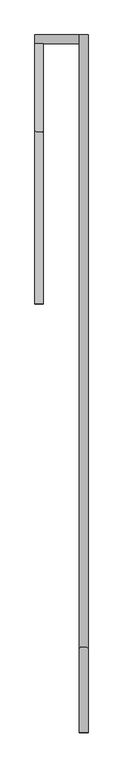
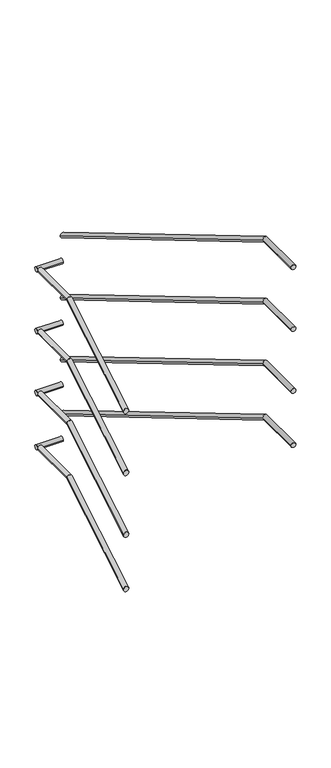
"""IFC4 building model written with IfcOpenShell, lengths in millimetres: railing geometry."""

import ifcopenshell
import ifcopenshell.guid

model = None  # the IFC model being written
_history = None  # IfcOwnerHistory: only IFC2X3 demands one
_inside = {}  # id of a spatial element -> (the spatial element, [elements in it])
_under = {}  # id of a project, library or spatial element -> (it, [spatial elements below it])
_declared = {}  # id of a project -> (the project, [libraries it declares])
_typed = {}  # id of a type object -> (the type object, [elements of that type])
_made_of = {}  # id of a material, layer set ... -> (it, [elements and type objects made of it])


def new_model(schema):
    """Start an empty IFC model of exactly this schema.

    Asked for "IFC4X3", IfcOpenShell would pick the latest addendum, in which some entities
    have other attributes; the version numbers below select the first issue.
    IFC2X3 requires an IfcOwnerHistory on every rooted entity: one is made here for all.
    """
    global model, _history
    if schema == "IFC4X3":
        model = ifcopenshell.file(schema_version=(4, 3, 0, 0))
    else:
        model = ifcopenshell.file(schema=schema)
    _inside.clear()
    _under.clear()
    _declared.clear()
    _typed.clear()
    _made_of.clear()
    _history = None
    if model.schema == "IFC2X3":
        org = make("IfcOrganization", Name="unknown")
        user = make(
            "IfcPersonAndOrganization",
            ThePerson=make("IfcPerson", FamilyName="unknown"),
            TheOrganization=org,
        )
        app = make(
            "IfcApplication",
            ApplicationDeveloper=org,
            Version="unknown",
            ApplicationFullName="unknown",
            ApplicationIdentifier="unknown",
        )
        _history = make(
            "IfcOwnerHistory",
            OwningUser=user,
            OwningApplication=app,
            ChangeAction="ADDED",
            CreationDate=0,
        )
    return model


def make(cls, **values):
    """One entity of the class cls with the attributes given. An attribute that is None is left unset."""
    return model.create_entity(
        cls, **{name: value for name, value in values.items() if value is not None}
    )


def rooted(cls, **values):
    """An entity with a GlobalId (a new one), such as an element, a storey or a relation."""
    return make(cls, GlobalId=ifcopenshell.guid.new(), OwnerHistory=_history, **values)


def si_unit(unit_type, name, prefix=None):
    """IfcSIUnit, for example si_unit("LENGTHUNIT", "METRE", prefix="MILLI")."""
    return make("IfcSIUnit", UnitType=unit_type, Prefix=prefix, Name=name)


def assignment(units):
    """IfcUnitAssignment: the units of a project."""
    return None if units is None else make("IfcUnitAssignment", Units=units)


def point(xyz):
    """IfcCartesianPoint."""
    return None if xyz is None else make("IfcCartesianPoint", Coordinates=xyz)


def direction(xyz):
    """IfcDirection."""
    return None if xyz is None else make("IfcDirection", DirectionRatios=xyz)


def frame(location, z_axis=None, x_axis=None):
    """IfcAxis2Placement3D, a coordinate frame: its origin and axes. An axis left out is left unset."""
    return make(
        "IfcAxis2Placement3D",
        Location=point(location),
        Axis=direction(z_axis),
        RefDirection=direction(x_axis),
    )


def origin():
    """The frame at (0, 0, 0) with its axes left unset."""
    return frame((0.0, 0.0, 0.0))


def place(relative_to, where):
    """IfcLocalPlacement: puts the frame where relative to a parent placement (None: the world)."""
    return make(
        "IfcLocalPlacement", PlacementRelTo=relative_to, RelativePlacement=where
    )


def context(
    kind, dimensions, precision=None, world=None, true_north=None, identifier=None
):
    """IfcGeometricRepresentationContext, for example the 3D "Model" context."""
    return make(
        "IfcGeometricRepresentationContext",
        ContextIdentifier=identifier,
        ContextType=kind,
        CoordinateSpaceDimension=dimensions,
        Precision=precision,
        WorldCoordinateSystem=world,
        TrueNorth=true_north,
    )


def project(units=None, contexts=None):
    """IfcProject with its units and contexts."""
    return rooted(
        "IfcProject",
        Name="project",
        RepresentationContexts=contexts,
        UnitsInContext=assignment(units),
    )


def spatial(cls, under=None, at=None, **own):
    """A site, building, storey or space (cls), placed at a placement, below another one or the project."""
    s = rooted(cls, ObjectPlacement=at, **own)
    if under is not None:
        _under.setdefault(under.id(), (under, []))[1].append(s)
    return s


def circle_curve(where, radius):
    """IfcCircle in the frame where."""
    return make("IfcCircle", Position=where, Radius=radius)


def ellipse_curve(where, semi_axis1, semi_axis2):
    """IfcEllipse in the frame where."""
    return make(
        "IfcEllipse", Position=where, SemiAxis1=semi_axis1, SemiAxis2=semi_axis2
    )


def shape(context_of_items, identifier, shape_type, items):
    """IfcShapeRepresentation: the items that make up one representation, for example the "Body"."""
    return make(
        "IfcShapeRepresentation",
        ContextOfItems=context_of_items,
        RepresentationIdentifier=identifier,
        RepresentationType=shape_type,
        Items=items,
    )


def source(mapping_origin, context_of_items, identifier, shape_type, items):
    """IfcRepresentationMap: a shape defined once, which mapped items show again and again."""
    return make(
        "IfcRepresentationMap",
        MappingOrigin=mapping_origin,
        MappedRepresentation=shape(context_of_items, identifier, shape_type, items),
    )


def transform(
    local_origin,
    x_axis=None,
    y_axis=None,
    z_axis=None,
    scale=None,
    scale2=None,
    scale3=None,
    uniform=True,
):
    """IfcCartesianTransformationOperator3D, or its non-uniform kind. x_axis, y_axis, z_axis: its Axis1, 2, 3."""
    if uniform:
        return make(
            "IfcCartesianTransformationOperator3D",
            Axis1=direction(x_axis),
            Axis2=direction(y_axis),
            LocalOrigin=point(local_origin),
            Scale=scale,
            Axis3=direction(z_axis),
        )
    return make(
        "IfcCartesianTransformationOperator3DnonUniform",
        Axis1=direction(x_axis),
        Axis2=direction(y_axis),
        LocalOrigin=point(local_origin),
        Scale=scale,
        Axis3=direction(z_axis),
        Scale2=scale2,
        Scale3=scale3,
    )


def mapped(mapping_source, mapping_target):
    """IfcMappedItem: shows the shape of a source again, moved by a transform."""
    return make(
        "IfcMappedItem", MappingSource=mapping_source, MappingTarget=mapping_target
    )


def made_of(thing, what):
    """Note that an element or type object is made of a material, layer set ...; save() writes the relation."""
    if what is not None:
        _made_of.setdefault(what.id(), (what, []))[1].append(thing)
    return thing


def element(
    cls,
    number,
    at=None,
    inside=None,
    cuts=None,
    type_object=None,
    material=None,
    context=None,
    identifier="Body",
    shape_type=None,
    held_by="IfcProductDefinitionShape",
    body=None,
    shapes=None,
    **own,
):
    """One element of the class cls, such as IfcWall. Its Tag is "e" and its number.

    at: its placement. inside: the storey or other place that contains it. cuts: it is an
    opening in that element (IfcRelVoidsElement). A single representation is given by context,
    identifier, shape_type and body (its items); several are given by shapes. held_by: the class
    of the entity that holds the representations. save() writes the other relations.
    """
    e = rooted(cls, Tag="e%d" % number, ObjectPlacement=at, **own)
    if body is not None:
        shapes = [shape(context, identifier, shape_type, body)]
    if shapes is not None:
        e.Representation = make(held_by, Representations=shapes)
    if inside is not None:
        _inside.setdefault(inside.id(), (inside, []))[1].append(e)
    if cuts is not None:
        rooted(
            "IfcRelVoidsElement", RelatingBuildingElement=cuts, RelatedOpeningElement=e
        )
    if type_object is not None:
        _typed.setdefault(type_object.id(), (type_object, []))[1].append(e)
    return made_of(e, material)


def aggregate(whole, parts):
    """IfcRelAggregates: a whole, such as a stair, and the parts it consists of."""
    return rooted("IfcRelAggregates", RelatingObject=whole, RelatedObjects=parts)


def save(model, path):
    """Write the relations noted so far, then the file.

    IfcRelAggregates (storeys below a building ...), IfcRelContainedInSpatialStructure (elements
    in a storey), IfcRelDefinesByType, IfcRelAssociatesMaterial and IfcRelDeclares: one each for
    every whole, place, type object, material and project.
    """
    for whole, parts in _under.values():
        aggregate(whole, parts)
    for where, things in _inside.values():
        rooted(
            "IfcRelContainedInSpatialStructure",
            RelatedElements=things,
            RelatingStructure=where,
        )
    for kind, things in _typed.values():
        rooted("IfcRelDefinesByType", RelatedObjects=things, RelatingType=kind)
    for what, things in _made_of.values():
        rooted("IfcRelAssociatesMaterial", RelatedObjects=things, RelatingMaterial=what)
    for by, libraries in _declared.values():
        rooted("IfcRelDeclares", RelatingContext=by, RelatedDefinitions=libraries)
    model.write(path)


def plane_surface(at):
    """IfcPlane: the flat surface through the origin of the frame at, square to its z axis."""
    return make("IfcPlane", Position=at)


def cylinder_surface(at, radius):
    """IfcCylindricalSurface: all points at the distance radius from the z axis of the frame at."""
    return make("IfcCylindricalSurface", Position=at, Radius=radius)


def advanced_brep(points, edges, surfaces, faces):
    """IfcAdvancedBrep: a solid bounded by faces that lie on surfaces and meet in shared edges.

    An edge is (start, end): straight between two places in points (the first is 0);
    or (start, end, curve); or (start, end, curve, False) where it runs against its curve.
    A face is (place in surfaces, loops), or (place, loops, False) where it looks against
    its surface's normal. A loop lists edges by number (the first is 1), with a minus sign
    where the edge is run from its end to its start. The first loop is the outer one.
    """
    corners = [point(p) for p in points]
    vertices = [make("IfcVertexPoint", VertexGeometry=c) for c in corners]
    made = []
    for start, end, *more in edges:
        made.append(
            make(
                "IfcEdgeCurve",
                EdgeStart=vertices[start],
                EdgeEnd=vertices[end],
                EdgeGeometry=more[0] if more else make("IfcPolyline", Points=[corners[start], corners[end]]),
                SameSense=more[1] if len(more) > 1 else True,
            )
        )
    hull = []
    for where, loops, *sense in faces:
        bounds = []
        for j, loop in enumerate(loops):
            ring = [make("IfcOrientedEdge", EdgeElement=made[abs(k) - 1], Orientation=k > 0) for k in loop]
            bounds.append(
                make(
                    "IfcFaceOuterBound" if j == 0 else "IfcFaceBound",
                    Bound=make("IfcEdgeLoop", EdgeList=ring),
                    Orientation=True,
                )
            )
        hull.append(make("IfcAdvancedFace", Bounds=bounds, FaceSurface=surfaces[where], SameSense=sense[0] if sense else True))
    return make("IfcAdvancedBrep", Outer=make("IfcClosedShell", CfsFaces=hull))


def railing_415aae61(model_context):
    return source(origin(), model_context, "Body", "AdvancedBrep", [
        advanced_brep(
        [(52769.6, 14329.5208589, 10810.697424), (52799.6, 14329.5208589, 10810.697424), (52769.6, 14933.6395577, 11169.5073179), (52799.6, 14933.6395577, 11169.5073179), (52769.6, 15239.9208589, 11169.5073179), (52799.6, 15239.9208589, 11169.5073179)],
        [
            (0, 1, ellipse_curve(frame((52784.6, 14329.5208589, 10810.697424), z_axis=(0.0, -1.0, 0.0), x_axis=(0.0, 0.0, -1.0)), 17.4462575, 15.0)),
            (1, 0, ellipse_curve(frame((52784.6, 14329.5208589, 10810.697424), z_axis=(0.0, -1.0, 0.0), x_axis=(0.0, 0.0, -1.0)), 17.4462575, 15.0)),
            (0, 2),
            (2, 3, ellipse_curve(frame((52784.6, 14933.6395577, 11169.5073179), z_axis=(0.0, -0.9643088850075937, -0.26477986006381166), x_axis=(0.0, 0.2647798600638126, -0.9643088850075935)), 15.5551818, 15.0)),
            (3, 1),
            (3, 2, ellipse_curve(frame((52784.6, 14933.6395577, 11169.5073179), z_axis=(0.0, -0.9643088850075937, -0.26477986006381166), x_axis=(0.0, 0.2647798600638126, -0.9643088850075935)), 15.5551818, 15.0)),
            (4, 5, circle_curve(frame((52784.6, 15239.9208589, 11169.5073179), z_axis=(0.0, 1.0, 0.0), x_axis=(1.0, 0.0, 0.0)), 15.0)),
            (5, 4, circle_curve(frame((52784.6, 15239.9208589, 11169.5073179), z_axis=(0.0, 1.0, 0.0), x_axis=(1.0, 0.0, 0.0)), 15.0)),
            (2, 4),
            (5, 3),
        ],
        [
            plane_surface(frame((52784.6, 14329.5208589, 10828.1436815), z_axis=(0.0, -1.0, 0.0), x_axis=(0.0, 0.0, 1.0))),
            cylinder_surface(frame((52784.6, 14337.180746, 10815.2469328), z_axis=(0.0, -0.8597832514091767, -0.5106591432612018), x_axis=(1.0, 0.0, 0.0)), 15.0),
            plane_surface(frame((52784.6, 15239.9208589, 11184.5073179), z_axis=(0.0, 1.0, 0.0), x_axis=(0.0, 0.0, 1.0))),
            cylinder_surface(frame((52784.6, 14929.5208589, 11169.5073179), z_axis=(0.0, -1.0, 0.0), x_axis=(1.0, 0.0, 0.0)), 15.0),
        ],
        [
            (0, [[1, 2]]),
            (1, [[-1, 3, 4, 5]]),
            (1, [[-2, -5, 6, -3]]),
            (2, [[7, 8]]),
            (3, [[-4, 9, -8, 10]]),
            (3, [[-6, -10, -7, -9]]),
        ],
    ),
        advanced_brep(
        [(52769.6, 15269.9208589, 11169.5073179), (52769.6, 15239.9208589, 11169.5073179), (52925.4, 15269.9208589, 11169.5073179), (52925.4, 15239.9208589, 11169.5073179)],
        [
            (0, 1, circle_curve(frame((52769.6, 15254.9208589, 11169.5073179), z_axis=(-1.0, 0.0, 0.0), x_axis=(0.0, -1.0, 0.0)), 15.0)),
            (1, 0, circle_curve(frame((52769.6, 15254.9208589, 11169.5073179), z_axis=(-1.0, 0.0, 0.0), x_axis=(0.0, -1.0, 0.0)), 15.0)),
            (2, 3, circle_curve(frame((52925.4, 15254.9208589, 11169.5073179), z_axis=(1.0, 0.0, 0.0), x_axis=(0.0, -1.0, 0.0)), 15.0)),
            (3, 2, circle_curve(frame((52925.4, 15254.9208589, 11169.5073179), z_axis=(1.0, 0.0, 0.0), x_axis=(0.0, -1.0, 0.0)), 15.0)),
            (0, 2),
            (3, 1),
        ],
        [
            plane_surface(frame((52769.6, 15254.9208589, 11184.5073179), z_axis=(-1.0, 0.0, 0.0), x_axis=(0.0, 1.0, 0.0))),
            plane_surface(frame((52925.4, 15254.9208589, 11184.5073179), z_axis=(1.0, 0.0, 0.0), x_axis=(0.0, 1.0, 0.0))),
            cylinder_surface(frame((52769.6, 15254.9208589, 11169.5073179), z_axis=(-1.0, 0.0, 0.0), x_axis=(0.0, -1.0, 0.0)), 15.0),
        ],
        [
            (0, [[1, 2]]),
            (1, [[3, 4]]),
            (2, [[-1, 5, -4, 6]]),
            (2, [[-2, -6, -3, -5]]),
        ],
    ),
        advanced_brep(
        [(52955.4, 15269.9208589, 11321.2477271), (52925.4, 15269.9208589, 11321.2477271), (52955.4, 13125.40216, 12594.9618634), (52925.4, 13125.40216, 12594.9618634), (52955.4, 12829.5208589, 12594.9618634), (52925.4, 12829.5208589, 12594.9618634)],
        [
            (0, 1, ellipse_curve(frame((52940.4, 15269.9208589, 11321.2477271), z_axis=(0.0, 1.0, 0.0), x_axis=(0.0, 0.0, -1.0)), 17.4462575, 15.0)),
            (1, 0, ellipse_curve(frame((52940.4, 15269.9208589, 11321.2477271), z_axis=(0.0, 1.0, 0.0), x_axis=(0.0, 0.0, -1.0)), 17.4462575, 15.0)),
            (0, 2),
            (2, 3, ellipse_curve(frame((52940.4, 13125.40216, 12594.9618634), z_axis=(0.0, 0.9643088850075937, -0.26477986006381166), x_axis=(0.0, -0.2647798600638126, -0.9643088850075935)), 15.5551818, 15.0)),
            (3, 1),
            (3, 2, ellipse_curve(frame((52940.4, 13125.40216, 12594.9618634), z_axis=(0.0, 0.9643088850075937, -0.26477986006381166), x_axis=(0.0, -0.2647798600638126, -0.9643088850075935)), 15.5551818, 15.0)),
            (4, 5, circle_curve(frame((52940.4, 12829.5208589, 12594.9618634), z_axis=(0.0, -1.0, 0.0), x_axis=(-1.0, 0.0, 0.0)), 15.0)),
            (5, 4, circle_curve(frame((52940.4, 12829.5208589, 12594.9618634), z_axis=(0.0, -1.0, 0.0), x_axis=(-1.0, 0.0, 0.0)), 15.0)),
            (2, 4),
            (5, 3),
        ],
        [
            plane_surface(frame((52940.4, 15269.9208589, 11338.6939846), z_axis=(0.0, 1.0, 0.0), x_axis=(0.0, 0.0, -1.0))),
            cylinder_surface(frame((52940.4, 15262.2609717, 11325.7972358), z_axis=(0.0, 0.8597832514091767, -0.5106591432612018), x_axis=(-1.0, 0.0, 0.0)), 15.0),
            plane_surface(frame((52940.4, 12829.5208589, 12609.9618634), z_axis=(0.0, -1.0, 0.0), x_axis=(0.0, 0.0, -1.0))),
            cylinder_surface(frame((52940.4, 13129.5208589, 12594.9618634), z_axis=(0.0, 1.0, 0.0), x_axis=(-1.0, 0.0, 0.0)), 15.0),
        ],
        [
            (0, [[1, 2]]),
            (1, [[-1, 3, 4, 5]]),
            (1, [[-2, -5, 6, -3]]),
            (2, [[7, 8]]),
            (3, [[-4, 9, -8, 10]]),
            (3, [[-6, -10, -7, -9]]),
        ],
    ),
        advanced_brep(
        [(52769.6, 14329.5208589, 10010.697424), (52799.6, 14329.5208589, 10010.697424), (52769.6, 14933.6395577, 10369.5073179), (52799.6, 14933.6395577, 10369.5073179), (52769.6, 15239.9208589, 10369.5073179), (52799.6, 15239.9208589, 10369.5073179)],
        [
            (0, 1, ellipse_curve(frame((52784.6, 14329.5208589, 10010.697424), z_axis=(0.0, -1.0, 0.0), x_axis=(0.0, 0.0, -1.0)), 17.4462575, 15.0)),
            (1, 0, ellipse_curve(frame((52784.6, 14329.5208589, 10010.697424), z_axis=(0.0, -1.0, 0.0), x_axis=(0.0, 0.0, -1.0)), 17.4462575, 15.0)),
            (0, 2),
            (2, 3, ellipse_curve(frame((52784.6, 14933.6395577, 10369.5073179), z_axis=(0.0, -0.9643088850075937, -0.26477986006381166), x_axis=(0.0, 0.2647798600638126, -0.9643088850075935)), 15.5551818, 15.0)),
            (3, 1),
            (3, 2, ellipse_curve(frame((52784.6, 14933.6395577, 10369.5073179), z_axis=(0.0, -0.9643088850075937, -0.26477986006381166), x_axis=(0.0, 0.2647798600638126, -0.9643088850075935)), 15.5551818, 15.0)),
            (4, 5, circle_curve(frame((52784.6, 15239.9208589, 10369.5073179), z_axis=(0.0, 1.0, 0.0), x_axis=(1.0, 0.0, 0.0)), 15.0)),
            (5, 4, circle_curve(frame((52784.6, 15239.9208589, 10369.5073179), z_axis=(0.0, 1.0, 0.0), x_axis=(1.0, 0.0, 0.0)), 15.0)),
            (2, 4),
            (5, 3),
        ],
        [
            plane_surface(frame((52784.6, 14329.5208589, 10028.1436815), z_axis=(0.0, -1.0, 0.0), x_axis=(0.0, 0.0, 1.0))),
            cylinder_surface(frame((52784.6, 14337.180746, 10015.2469328), z_axis=(0.0, -0.8597832514091767, -0.5106591432612018), x_axis=(1.0, 0.0, 0.0)), 15.0),
            plane_surface(frame((52784.6, 15239.9208589, 10384.5073179), z_axis=(0.0, 1.0, 0.0), x_axis=(0.0, 0.0, 1.0))),
            cylinder_surface(frame((52784.6, 14929.5208589, 10369.5073179), z_axis=(0.0, -1.0, 0.0), x_axis=(1.0, 0.0, 0.0)), 15.0),
        ],
        [
            (0, [[1, 2]]),
            (1, [[-1, 3, 4, 5]]),
            (1, [[-2, -5, 6, -3]]),
            (2, [[7, 8]]),
            (3, [[-4, 9, -8, 10]]),
            (3, [[-6, -10, -7, -9]]),
        ],
    ),
        advanced_brep(
        [(52769.6, 15269.9208589, 10369.5073179), (52769.6, 15239.9208589, 10369.5073179), (52925.4, 15269.9208589, 10369.5073179), (52925.4, 15239.9208589, 10369.5073179)],
        [
            (0, 1, circle_curve(frame((52769.6, 15254.9208589, 10369.5073179), z_axis=(-1.0, 0.0, 0.0), x_axis=(0.0, -1.0, 0.0)), 15.0)),
            (1, 0, circle_curve(frame((52769.6, 15254.9208589, 10369.5073179), z_axis=(-1.0, 0.0, 0.0), x_axis=(0.0, -1.0, 0.0)), 15.0)),
            (2, 3, circle_curve(frame((52925.4, 15254.9208589, 10369.5073179), z_axis=(1.0, 0.0, 0.0), x_axis=(0.0, -1.0, 0.0)), 15.0)),
            (3, 2, circle_curve(frame((52925.4, 15254.9208589, 10369.5073179), z_axis=(1.0, 0.0, 0.0), x_axis=(0.0, -1.0, 0.0)), 15.0)),
            (0, 2),
            (3, 1),
        ],
        [
            plane_surface(frame((52769.6, 15254.9208589, 10384.5073179), z_axis=(-1.0, 0.0, 0.0), x_axis=(0.0, 1.0, 0.0))),
            plane_surface(frame((52925.4, 15254.9208589, 10384.5073179), z_axis=(1.0, 0.0, 0.0), x_axis=(0.0, 1.0, 0.0))),
            cylinder_surface(frame((52769.6, 15254.9208589, 10369.5073179), z_axis=(-1.0, 0.0, 0.0), x_axis=(0.0, -1.0, 0.0)), 15.0),
        ],
        [
            (0, [[1, 2]]),
            (1, [[3, 4]]),
            (2, [[-1, 5, -4, 6]]),
            (2, [[-2, -6, -3, -5]]),
        ],
    ),
        advanced_brep(
        [(52955.4, 15269.9208589, 10521.2477271), (52925.4, 15269.9208589, 10521.2477271), (52955.4, 13125.40216, 11794.9618634), (52925.4, 13125.40216, 11794.9618634), (52955.4, 12829.5208589, 11794.9618634), (52925.4, 12829.5208589, 11794.9618634)],
        [
            (0, 1, ellipse_curve(frame((52940.4, 15269.9208589, 10521.2477271), z_axis=(0.0, 1.0, 0.0), x_axis=(0.0, 0.0, -1.0)), 17.4462575, 15.0)),
            (1, 0, ellipse_curve(frame((52940.4, 15269.9208589, 10521.2477271), z_axis=(0.0, 1.0, 0.0), x_axis=(0.0, 0.0, -1.0)), 17.4462575, 15.0)),
            (0, 2),
            (2, 3, ellipse_curve(frame((52940.4, 13125.40216, 11794.9618634), z_axis=(0.0, 0.9643088850075937, -0.26477986006381166), x_axis=(0.0, -0.2647798600638126, -0.9643088850075935)), 15.5551818, 15.0)),
            (3, 1),
            (3, 2, ellipse_curve(frame((52940.4, 13125.40216, 11794.9618634), z_axis=(0.0, 0.9643088850075937, -0.26477986006381166), x_axis=(0.0, -0.2647798600638126, -0.9643088850075935)), 15.5551818, 15.0)),
            (4, 5, circle_curve(frame((52940.4, 12829.5208589, 11794.9618634), z_axis=(0.0, -1.0, 0.0), x_axis=(-1.0, 0.0, 0.0)), 15.0)),
            (5, 4, circle_curve(frame((52940.4, 12829.5208589, 11794.9618634), z_axis=(0.0, -1.0, 0.0), x_axis=(-1.0, 0.0, 0.0)), 15.0)),
            (2, 4),
            (5, 3),
        ],
        [
            plane_surface(frame((52940.4, 15269.9208589, 10538.6939846), z_axis=(0.0, 1.0, 0.0), x_axis=(0.0, 0.0, -1.0))),
            cylinder_surface(frame((52940.4, 15262.2609717, 10525.7972358), z_axis=(0.0, 0.8597832514091767, -0.5106591432612018), x_axis=(-1.0, 0.0, 0.0)), 15.0),
            plane_surface(frame((52940.4, 12829.5208589, 11809.9618634), z_axis=(0.0, -1.0, 0.0), x_axis=(0.0, 0.0, -1.0))),
            cylinder_surface(frame((52940.4, 13129.5208589, 11794.9618634), z_axis=(0.0, 1.0, 0.0), x_axis=(-1.0, 0.0, 0.0)), 15.0),
        ],
        [
            (0, [[1, 2]]),
            (1, [[-1, 3, 4, 5]]),
            (1, [[-2, -5, 6, -3]]),
            (2, [[7, 8]]),
            (3, [[-4, 9, -8, 10]]),
            (3, [[-6, -10, -7, -9]]),
        ],
    ),
        advanced_brep(
        [(52769.6, 14329.5208589, 10410.697424), (52799.6, 14329.5208589, 10410.697424), (52769.6, 14933.6395577, 10769.5073179), (52799.6, 14933.6395577, 10769.5073179), (52769.6, 15239.9208589, 10769.5073179), (52799.6, 15239.9208589, 10769.5073179)],
        [
            (0, 1, ellipse_curve(frame((52784.6, 14329.5208589, 10410.697424), z_axis=(0.0, -1.0, 0.0), x_axis=(0.0, 0.0, -1.0)), 17.4462575, 15.0)),
            (1, 0, ellipse_curve(frame((52784.6, 14329.5208589, 10410.697424), z_axis=(0.0, -1.0, 0.0), x_axis=(0.0, 0.0, -1.0)), 17.4462575, 15.0)),
            (0, 2),
            (2, 3, ellipse_curve(frame((52784.6, 14933.6395577, 10769.5073179), z_axis=(0.0, -0.9643088850075937, -0.26477986006381166), x_axis=(0.0, 0.2647798600638126, -0.9643088850075935)), 15.5551818, 15.0)),
            (3, 1),
            (3, 2, ellipse_curve(frame((52784.6, 14933.6395577, 10769.5073179), z_axis=(0.0, -0.9643088850075937, -0.26477986006381166), x_axis=(0.0, 0.2647798600638126, -0.9643088850075935)), 15.5551818, 15.0)),
            (4, 5, circle_curve(frame((52784.6, 15239.9208589, 10769.5073179), z_axis=(0.0, 1.0, 0.0), x_axis=(1.0, 0.0, 0.0)), 15.0)),
            (5, 4, circle_curve(frame((52784.6, 15239.9208589, 10769.5073179), z_axis=(0.0, 1.0, 0.0), x_axis=(1.0, 0.0, 0.0)), 15.0)),
            (2, 4),
            (5, 3),
        ],
        [
            plane_surface(frame((52784.6, 14329.5208589, 10428.1436815), z_axis=(0.0, -1.0, 0.0), x_axis=(0.0, 0.0, 1.0))),
            cylinder_surface(frame((52784.6, 14337.180746, 10415.2469328), z_axis=(0.0, -0.8597832514091767, -0.5106591432612018), x_axis=(1.0, 0.0, 0.0)), 15.0),
            plane_surface(frame((52784.6, 15239.9208589, 10784.5073179), z_axis=(0.0, 1.0, 0.0), x_axis=(0.0, 0.0, 1.0))),
            cylinder_surface(frame((52784.6, 14929.5208589, 10769.5073179), z_axis=(0.0, -1.0, 0.0), x_axis=(1.0, 0.0, 0.0)), 15.0),
        ],
        [
            (0, [[1, 2]]),
            (1, [[-1, 3, 4, 5]]),
            (1, [[-2, -5, 6, -3]]),
            (2, [[7, 8]]),
            (3, [[-4, 9, -8, 10]]),
            (3, [[-6, -10, -7, -9]]),
        ],
    ),
        advanced_brep(
        [(52769.6, 15269.9208589, 10769.5073179), (52769.6, 15239.9208589, 10769.5073179), (52925.4, 15269.9208589, 10769.5073179), (52925.4, 15239.9208589, 10769.5073179)],
        [
            (0, 1, circle_curve(frame((52769.6, 15254.9208589, 10769.5073179), z_axis=(-1.0, 0.0, 0.0), x_axis=(0.0, -1.0, 0.0)), 15.0)),
            (1, 0, circle_curve(frame((52769.6, 15254.9208589, 10769.5073179), z_axis=(-1.0, 0.0, 0.0), x_axis=(0.0, -1.0, 0.0)), 15.0)),
            (2, 3, circle_curve(frame((52925.4, 15254.9208589, 10769.5073179), z_axis=(1.0, 0.0, 0.0), x_axis=(0.0, -1.0, 0.0)), 15.0)),
            (3, 2, circle_curve(frame((52925.4, 15254.9208589, 10769.5073179), z_axis=(1.0, 0.0, 0.0), x_axis=(0.0, -1.0, 0.0)), 15.0)),
            (0, 2),
            (3, 1),
        ],
        [
            plane_surface(frame((52769.6, 15254.9208589, 10784.5073179), z_axis=(-1.0, 0.0, 0.0), x_axis=(0.0, 1.0, 0.0))),
            plane_surface(frame((52925.4, 15254.9208589, 10784.5073179), z_axis=(1.0, 0.0, 0.0), x_axis=(0.0, 1.0, 0.0))),
            cylinder_surface(frame((52769.6, 15254.9208589, 10769.5073179), z_axis=(-1.0, 0.0, 0.0), x_axis=(0.0, -1.0, 0.0)), 15.0),
        ],
        [
            (0, [[1, 2]]),
            (1, [[3, 4]]),
            (2, [[-1, 5, -4, 6]]),
            (2, [[-2, -6, -3, -5]]),
        ],
    ),
        advanced_brep(
        [(52955.4, 15269.9208589, 10921.2477271), (52925.4, 15269.9208589, 10921.2477271), (52955.4, 13125.40216, 12194.9618634), (52925.4, 13125.40216, 12194.9618634), (52955.4, 12829.5208589, 12194.9618634), (52925.4, 12829.5208589, 12194.9618634)],
        [
            (0, 1, ellipse_curve(frame((52940.4, 15269.9208589, 10921.2477271), z_axis=(0.0, 1.0, 0.0), x_axis=(0.0, 0.0, -1.0)), 17.4462575, 15.0)),
            (1, 0, ellipse_curve(frame((52940.4, 15269.9208589, 10921.2477271), z_axis=(0.0, 1.0, 0.0), x_axis=(0.0, 0.0, -1.0)), 17.4462575, 15.0)),
            (0, 2),
            (2, 3, ellipse_curve(frame((52940.4, 13125.40216, 12194.9618634), z_axis=(0.0, 0.9643088850075937, -0.26477986006381166), x_axis=(0.0, -0.2647798600638126, -0.9643088850075935)), 15.5551818, 15.0)),
            (3, 1),
            (3, 2, ellipse_curve(frame((52940.4, 13125.40216, 12194.9618634), z_axis=(0.0, 0.9643088850075937, -0.26477986006381166), x_axis=(0.0, -0.2647798600638126, -0.9643088850075935)), 15.5551818, 15.0)),
            (4, 5, circle_curve(frame((52940.4, 12829.5208589, 12194.9618634), z_axis=(0.0, -1.0, 0.0), x_axis=(-1.0, 0.0, 0.0)), 15.0)),
            (5, 4, circle_curve(frame((52940.4, 12829.5208589, 12194.9618634), z_axis=(0.0, -1.0, 0.0), x_axis=(-1.0, 0.0, 0.0)), 15.0)),
            (2, 4),
            (5, 3),
        ],
        [
            plane_surface(frame((52940.4, 15269.9208589, 10938.6939846), z_axis=(0.0, 1.0, 0.0), x_axis=(0.0, 0.0, -1.0))),
            cylinder_surface(frame((52940.4, 15262.2609717, 10925.7972358), z_axis=(0.0, 0.8597832514091767, -0.5106591432612018), x_axis=(-1.0, 0.0, 0.0)), 15.0),
            plane_surface(frame((52940.4, 12829.5208589, 12209.9618634), z_axis=(0.0, -1.0, 0.0), x_axis=(0.0, 0.0, -1.0))),
            cylinder_surface(frame((52940.4, 13129.5208589, 12194.9618634), z_axis=(0.0, 1.0, 0.0), x_axis=(-1.0, 0.0, 0.0)), 15.0),
        ],
        [
            (0, [[1, 2]]),
            (1, [[-1, 3, 4, 5]]),
            (1, [[-2, -5, 6, -3]]),
            (2, [[7, 8]]),
            (3, [[-4, 9, -8, 10]]),
            (3, [[-6, -10, -7, -9]]),
        ],
    ),
        advanced_brep(
        [(52769.6, 14329.5208589, 9660.697424), (52799.6, 14329.5208589, 9660.697424), (52769.6, 14933.6395577, 10019.5073179), (52799.6, 14933.6395577, 10019.5073179), (52769.6, 15239.9208589, 10019.5073179), (52799.6, 15239.9208589, 10019.5073179)],
        [
            (0, 1, ellipse_curve(frame((52784.6, 14329.5208589, 9660.697424), z_axis=(0.0, -1.0, 0.0), x_axis=(0.0, 0.0, -1.0)), 17.4462575, 15.0)),
            (1, 0, ellipse_curve(frame((52784.6, 14329.5208589, 9660.697424), z_axis=(0.0, -1.0, 0.0), x_axis=(0.0, 0.0, -1.0)), 17.4462575, 15.0)),
            (0, 2),
            (2, 3, ellipse_curve(frame((52784.6, 14933.6395577, 10019.5073179), z_axis=(0.0, -0.9643088850075937, -0.26477986006381166), x_axis=(0.0, 0.2647798600638126, -0.9643088850075935)), 15.5551818, 15.0)),
            (3, 1),
            (3, 2, ellipse_curve(frame((52784.6, 14933.6395577, 10019.5073179), z_axis=(0.0, -0.9643088850075937, -0.26477986006381166), x_axis=(0.0, 0.2647798600638126, -0.9643088850075935)), 15.5551818, 15.0)),
            (4, 5, circle_curve(frame((52784.6, 15239.9208589, 10019.5073179), z_axis=(0.0, 1.0, 0.0), x_axis=(1.0, 0.0, 0.0)), 15.0)),
            (5, 4, circle_curve(frame((52784.6, 15239.9208589, 10019.5073179), z_axis=(0.0, 1.0, 0.0), x_axis=(1.0, 0.0, 0.0)), 15.0)),
            (2, 4),
            (5, 3),
        ],
        [
            plane_surface(frame((52784.6, 14329.5208589, 9678.1436815), z_axis=(0.0, -1.0, 0.0), x_axis=(0.0, 0.0, 1.0))),
            cylinder_surface(frame((52784.6, 14337.180746, 9665.2469328), z_axis=(0.0, -0.8597832514091767, -0.5106591432612018), x_axis=(1.0, 0.0, 0.0)), 15.0),
            plane_surface(frame((52784.6, 15239.9208589, 10034.5073179), z_axis=(0.0, 1.0, 0.0), x_axis=(0.0, 0.0, 1.0))),
            cylinder_surface(frame((52784.6, 14929.5208589, 10019.5073179), z_axis=(0.0, -1.0, 0.0), x_axis=(1.0, 0.0, 0.0)), 15.0),
        ],
        [
            (0, [[1, 2]]),
            (1, [[-1, 3, 4, 5]]),
            (1, [[-2, -5, 6, -3]]),
            (2, [[7, 8]]),
            (3, [[-4, 9, -8, 10]]),
            (3, [[-6, -10, -7, -9]]),
        ],
    ),
        advanced_brep(
        [(52769.6, 15269.9208589, 10019.5073179), (52769.6, 15239.9208589, 10019.5073179), (52925.4, 15269.9208589, 10019.5073179), (52925.4, 15239.9208589, 10019.5073179)],
        [
            (0, 1, circle_curve(frame((52769.6, 15254.9208589, 10019.5073179), z_axis=(-1.0, 0.0, 0.0), x_axis=(0.0, -1.0, 0.0)), 15.0)),
            (1, 0, circle_curve(frame((52769.6, 15254.9208589, 10019.5073179), z_axis=(-1.0, 0.0, 0.0), x_axis=(0.0, -1.0, 0.0)), 15.0)),
            (2, 3, circle_curve(frame((52925.4, 15254.9208589, 10019.5073179), z_axis=(1.0, 0.0, 0.0), x_axis=(0.0, -1.0, 0.0)), 15.0)),
            (3, 2, circle_curve(frame((52925.4, 15254.9208589, 10019.5073179), z_axis=(1.0, 0.0, 0.0), x_axis=(0.0, -1.0, 0.0)), 15.0)),
            (0, 2),
            (3, 1),
        ],
        [
            plane_surface(frame((52769.6, 15254.9208589, 10034.5073179), z_axis=(-1.0, 0.0, 0.0), x_axis=(0.0, 1.0, 0.0))),
            plane_surface(frame((52925.4, 15254.9208589, 10034.5073179), z_axis=(1.0, 0.0, 0.0), x_axis=(0.0, 1.0, 0.0))),
            cylinder_surface(frame((52769.6, 15254.9208589, 10019.5073179), z_axis=(-1.0, 0.0, 0.0), x_axis=(0.0, -1.0, 0.0)), 15.0),
        ],
        [
            (0, [[1, 2]]),
            (1, [[3, 4]]),
            (2, [[-1, 5, -4, 6]]),
            (2, [[-2, -6, -3, -5]]),
        ],
    ),
        advanced_brep(
        [(52955.4, 15269.9208589, 10171.2477271), (52925.4, 15269.9208589, 10171.2477271), (52955.4, 13125.40216, 11444.9618634), (52925.4, 13125.40216, 11444.9618634), (52955.4, 12829.5208589, 11444.9618634), (52925.4, 12829.5208589, 11444.9618634)],
        [
            (0, 1, ellipse_curve(frame((52940.4, 15269.9208589, 10171.2477271), z_axis=(0.0, 1.0, 0.0), x_axis=(0.0, 0.0, -1.0)), 17.4462575, 15.0)),
            (1, 0, ellipse_curve(frame((52940.4, 15269.9208589, 10171.2477271), z_axis=(0.0, 1.0, 0.0), x_axis=(0.0, 0.0, -1.0)), 17.4462575, 15.0)),
            (0, 2),
            (2, 3, ellipse_curve(frame((52940.4, 13125.40216, 11444.9618634), z_axis=(0.0, 0.9643088850075937, -0.26477986006381166), x_axis=(0.0, -0.2647798600638126, -0.9643088850075935)), 15.5551818, 15.0)),
            (3, 1),
            (3, 2, ellipse_curve(frame((52940.4, 13125.40216, 11444.9618634), z_axis=(0.0, 0.9643088850075937, -0.26477986006381166), x_axis=(0.0, -0.2647798600638126, -0.9643088850075935)), 15.5551818, 15.0)),
            (4, 5, circle_curve(frame((52940.4, 12829.5208589, 11444.9618634), z_axis=(0.0, -1.0, 0.0), x_axis=(-1.0, 0.0, 0.0)), 15.0)),
            (5, 4, circle_curve(frame((52940.4, 12829.5208589, 11444.9618634), z_axis=(0.0, -1.0, 0.0), x_axis=(-1.0, 0.0, 0.0)), 15.0)),
            (2, 4),
            (5, 3),
        ],
        [
            plane_surface(frame((52940.4, 15269.9208589, 10188.6939846), z_axis=(0.0, 1.0, 0.0), x_axis=(0.0, 0.0, -1.0))),
            cylinder_surface(frame((52940.4, 15262.2609717, 10175.7972358), z_axis=(0.0, 0.8597832514091767, -0.5106591432612018), x_axis=(-1.0, 0.0, 0.0)), 15.0),
            plane_surface(frame((52940.4, 12829.5208589, 11459.9618634), z_axis=(0.0, -1.0, 0.0), x_axis=(0.0, 0.0, -1.0))),
            cylinder_surface(frame((52940.4, 13129.5208589, 11444.9618634), z_axis=(0.0, 1.0, 0.0), x_axis=(-1.0, 0.0, 0.0)), 15.0),
        ],
        [
            (0, [[1, 2]]),
            (1, [[-1, 3, 4, 5]]),
            (1, [[-2, -5, 6, -3]]),
            (2, [[7, 8]]),
            (3, [[-4, 9, -8, 10]]),
            (3, [[-6, -10, -7, -9]]),
        ],
    ),
    ])


if __name__ == "__main__":
    model = new_model("IFC4")
    model_context = context("Model", 3, world=origin())
    ifc_project = project(units=[si_unit("LENGTHUNIT", "METRE", prefix="MILLI")], contexts=[model_context])
    site = spatial("IfcSite", under=ifc_project)
    building = spatial("IfcBuilding", under=site)
    placement = place(None, origin())
    railing_shape = railing_415aae61(model_context)
    element("IfcRailing", 1, at=placement, inside=building, context=model_context, shape_type="MappedRepresentation", body=[
        mapped(railing_shape, transform((0.0, 0.0, 0.0), x_axis=(1.0, 0.0, 0.0), y_axis=(0.0, 1.0, 0.0), z_axis=(0.0, 0.0, 1.0))),
    ])
    save(model, "model.ifc")
